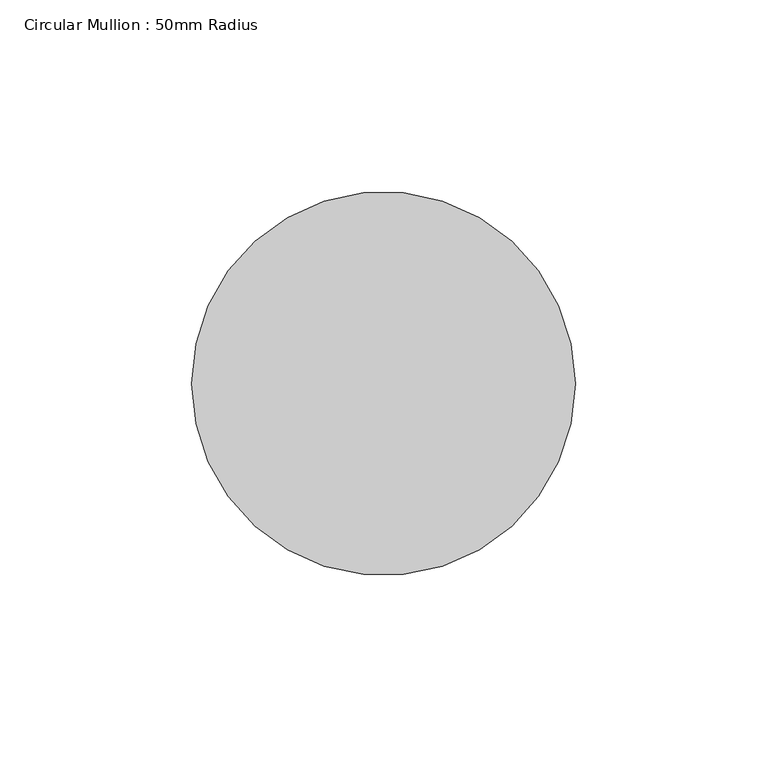
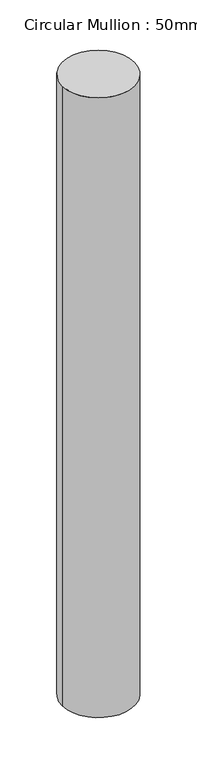
"""IFC4 building model written with IfcOpenShell, lengths in millimetres: member geometry, Circular Mullion : 50mm Radius."""

from ifc_helpers import new_model, si_unit, point, frame, origin, origin_2d, place, context, project, spatial, circle_curve, trimmed, segment, composite_curve, outline, extrude, source, transform, mapped, element, save


def circular_mullion_50mm_radius_121ef339(model_context):
    return source(origin(), model_context, "Body", "SweptSolid", [
        extrude(outline(composite_curve([segment(trimmed(circle_curve(origin_2d(), 50.0), [point((50.0, 0.0))], [point((-50.0, 0.0))], False, "CARTESIAN"), True, "CONTINUOUS"), segment(trimmed(circle_curve(origin_2d(), 50.0), [point((-50.0, 0.0))], [point((50.0, 0.0))], False, "CARTESIAN"), True, "CONTINUOUS")], self_intersect=False)), frame((0.0, 0.0, -909.9372285), z_axis=(0.0, 0.0, 1.0), x_axis=(1.0, 0.0, 0.0)), (0.0, 0.0, 1.0), 909.9372285),
    ])


if __name__ == "__main__":
    model = new_model("IFC4")
    model_context = context("Model", 3, world=origin())
    ifc_project = project(units=[si_unit("LENGTHUNIT", "METRE", prefix="MILLI")], contexts=[model_context])
    site = spatial("IfcSite", under=ifc_project)
    building = spatial("IfcBuilding", under=site)
    placement = place(None, origin())
    circular_mullion_50mm_radius_shape = circular_mullion_50mm_radius_121ef339(model_context)
    element("IfcMember", 1, ObjectType="Circular Mullion : 50mm Radius", at=placement, inside=building, context=model_context, shape_type="MappedRepresentation", body=[
        mapped(circular_mullion_50mm_radius_shape, transform((0.0, 0.0, 0.0), x_axis=(1.0, 0.0, 0.0), y_axis=(0.0, 1.0, 0.0), z_axis=(0.0, 0.0, 1.0))),
    ])
    save(model, "model.ifc")

# Revit data of these elements
# Type "Circular Mullion : 50mm Radius"
#   built-in parameter 1007350 = 0.164042 (stored number, unit not read)
# Element 1 (IfcMember, "Circular Mullion : 50mm Radius")
#   Materials on its faces: "Aluminium"
# Materials
#   "Aluminium": class "Metal", colour RGB 247 247 247, transparency 0, Description = "Aluminium 6061", Cost = 0
